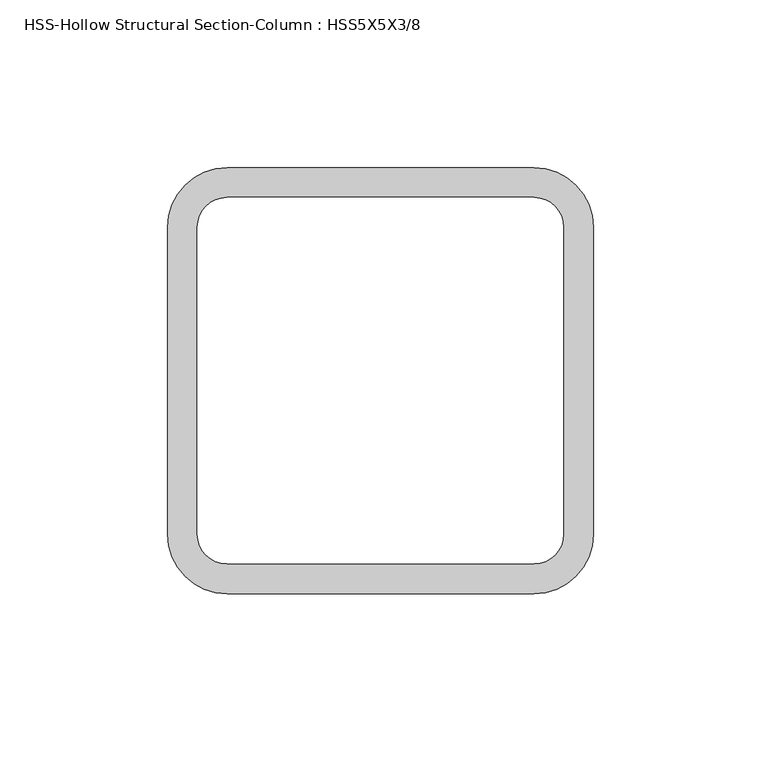
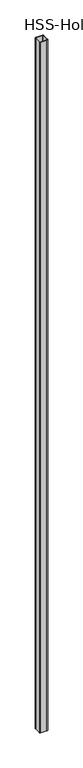
"""IFC4 building model written with IfcOpenShell, lengths in millimetres: column geometry, HSS-Hollow Structural Section-Column : HSS5X5X3/8."""

from ifc_helpers import new_model, si_unit, point, frame, frame_2d, origin, place, context, project, spatial, polyline, circle_curve, trimmed, segment, composite_curve, outline, extrude, source, transform, mapped, element, save


def hss_hollow_structural_section_column_hss5x5x3_8_a8b47676(model_context):
    return source(origin(), model_context, "Body", "SweptSolid", [
        extrude(outline(composite_curve([segment(trimmed(circle_curve(frame_2d((45.7708, 45.7708)), 17.7292), [point((45.7708, 63.5))], [point((63.5, 45.7708))], False, "CARTESIAN"), True, "CONTINUOUS"), segment(polyline([(63.5, 45.7708), (63.5, -45.7708)]), True, "CONTINUOUS"), segment(trimmed(circle_curve(frame_2d((45.7708, -45.7708)), 17.7292), [point((63.5, -45.7708))], [point((45.7708, -63.5))], False, "CARTESIAN"), True, "CONTINUOUS"), segment(polyline([(45.7708, -63.5), (-45.7708, -63.5)]), True, "CONTINUOUS"), segment(trimmed(circle_curve(frame_2d((-45.7708, -45.7708)), 17.7292), [point((-45.7708, -63.5))], [point((-63.5, -45.7708))], False, "CARTESIAN"), True, "CONTINUOUS"), segment(polyline([(-63.5, -45.7708), (-63.5, 45.7708)]), True, "CONTINUOUS"), segment(trimmed(circle_curve(frame_2d((-45.7708, 45.7708)), 17.7292), [point((-63.5, 45.7708))], [point((-45.7708, 63.5))], False, "CARTESIAN"), True, "CONTINUOUS"), segment(polyline([(-45.7708, 63.5), (45.7708, 63.5)]), True, "CONTINUOUS")], self_intersect=False), holes=[composite_curve([segment(polyline([(45.7708, 54.6354), (-45.7708, 54.6354)]), True, "CONTINUOUS"), segment(trimmed(circle_curve(frame_2d((-45.7708, 45.7708)), 8.8646), [point((-45.7708, 54.6354))], [point((-54.6354, 45.7708))], True, "CARTESIAN"), True, "CONTINUOUS"), segment(polyline([(-54.6354, 45.7708), (-54.6354, -45.7708)]), True, "CONTINUOUS"), segment(trimmed(circle_curve(frame_2d((-45.7708, -45.7708)), 8.8646), [point((-54.6354, -45.7708))], [point((-45.7708, -54.6354))], True, "CARTESIAN"), True, "CONTINUOUS"), segment(polyline([(-45.7708, -54.6354), (45.7708, -54.6354)]), True, "CONTINUOUS"), segment(trimmed(circle_curve(frame_2d((45.7708, -45.7708)), 8.8646), [point((45.7708, -54.6354))], [point((54.6354, -45.7708))], True, "CARTESIAN"), True, "CONTINUOUS"), segment(polyline([(54.6354, -45.7708), (54.6354, 45.7708)]), True, "CONTINUOUS"), segment(trimmed(circle_curve(frame_2d((45.7708, 45.7708)), 8.8646), [point((54.6354, 45.7708))], [point((45.7708, 54.6354))], True, "CARTESIAN"), True, "CONTINUOUS")], self_intersect=False)]), frame((0.0, 0.0, 16408.4), z_axis=(0.0, 0.0, 1.0), x_axis=(1.0, 0.0, 0.0)), (0.0, 0.0, 1.0), 11176.0),
    ])


if __name__ == "__main__":
    model = new_model("IFC4")
    model_context = context("Model", 3, world=origin())
    ifc_project = project(units=[si_unit("LENGTHUNIT", "METRE", prefix="MILLI")], contexts=[model_context])
    site = spatial("IfcSite", under=ifc_project)
    building = spatial("IfcBuilding", under=site)
    placement = place(None, origin())
    hss_hollow_structural_section_column_hss5x5x3_8_shape = hss_hollow_structural_section_column_hss5x5x3_8_a8b47676(model_context)
    element("IfcColumn", 1, ObjectType="HSS-Hollow Structural Section-Column : HSS5X5X3/8", at=placement, inside=building, context=model_context, shape_type="MappedRepresentation", body=[
        mapped(hss_hollow_structural_section_column_hss5x5x3_8_shape, transform((0.0, 0.0, 0.0), x_axis=(1.0, 0.0, 0.0), y_axis=(0.0, 1.0, 0.0), z_axis=(0.0, 0.0, 1.0))),
    ])
    save(model, "model.ifc")

# Revit data of these elements
# Type "HSS-Hollow Structural Section-Column : HSS5X5X3/8"
#   Assembly Code = "B10"
#   Shape = "Square"
#   W = 22.3
#   Ht = 0' - 5"
#   b = 0' - 5"
#   kr = 0' - 0.698"
#   t = 0' - 0.349"
#   A = 0.0429167 SF
#   Structural Material [instance default] = Steel ASTM A500, Grade B, Rectangular and Square
# Element 1 (IfcColumn, "HSS-Hollow Structural Section-Column : HSS5X5X3/8")
#   Materials on its faces: "Steel ASTM A500, Grade B, Rectangular and Square"
# Materials
#   "Steel ASTM A500, Grade B, Rectangular and Square": class "Metal", colour RGB 199 199 199, transparency 0, Description = "Carbon steel", Cost = 0
